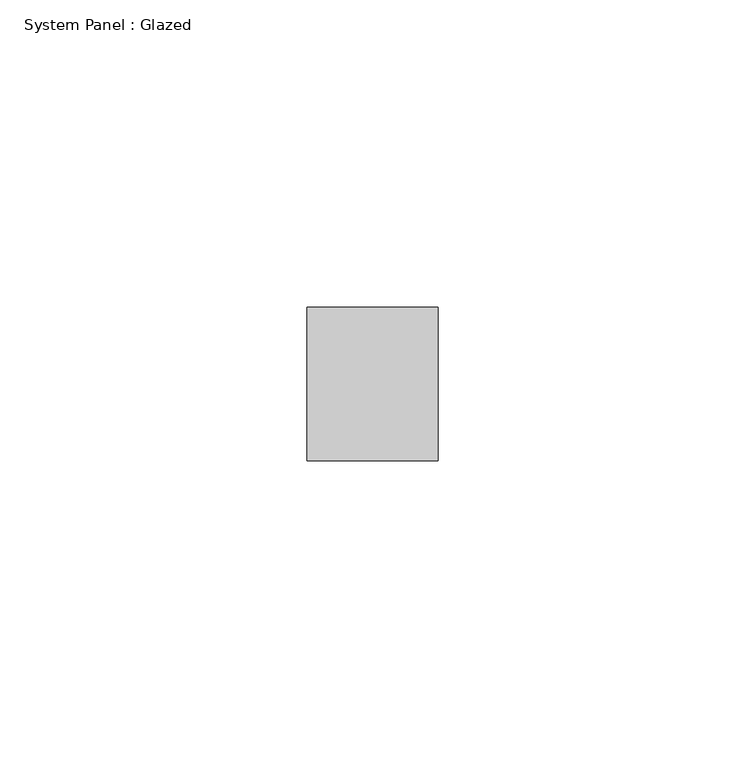
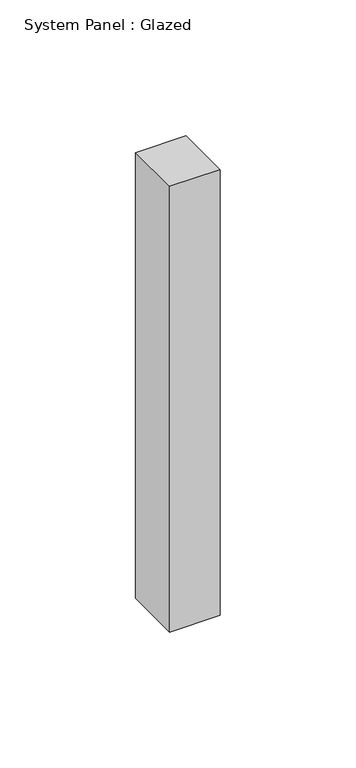
"""IFC4 building model written with IfcOpenShell, lengths in millimetres: plate geometry, System Panel : Glazed."""

import ifcopenshell
import ifcopenshell.guid

model = None  # the IFC model being written
_history = None  # IfcOwnerHistory: only IFC2X3 demands one
_inside = {}  # id of a spatial element -> (the spatial element, [elements in it])
_under = {}  # id of a project, library or spatial element -> (it, [spatial elements below it])
_declared = {}  # id of a project -> (the project, [libraries it declares])
_typed = {}  # id of a type object -> (the type object, [elements of that type])
_made_of = {}  # id of a material, layer set ... -> (it, [elements and type objects made of it])


def new_model(schema):
    """Start an empty IFC model of exactly this schema.

    Asked for "IFC4X3", IfcOpenShell would pick the latest addendum, in which some entities
    have other attributes; the version numbers below select the first issue.
    IFC2X3 requires an IfcOwnerHistory on every rooted entity: one is made here for all.
    """
    global model, _history
    if schema == "IFC4X3":
        model = ifcopenshell.file(schema_version=(4, 3, 0, 0))
    else:
        model = ifcopenshell.file(schema=schema)
    _inside.clear()
    _under.clear()
    _declared.clear()
    _typed.clear()
    _made_of.clear()
    _history = None
    if model.schema == "IFC2X3":
        org = make("IfcOrganization", Name="unknown")
        user = make(
            "IfcPersonAndOrganization",
            ThePerson=make("IfcPerson", FamilyName="unknown"),
            TheOrganization=org,
        )
        app = make(
            "IfcApplication",
            ApplicationDeveloper=org,
            Version="unknown",
            ApplicationFullName="unknown",
            ApplicationIdentifier="unknown",
        )
        _history = make(
            "IfcOwnerHistory",
            OwningUser=user,
            OwningApplication=app,
            ChangeAction="ADDED",
            CreationDate=0,
        )
    return model


def make(cls, **values):
    """One entity of the class cls with the attributes given. An attribute that is None is left unset."""
    return model.create_entity(
        cls, **{name: value for name, value in values.items() if value is not None}
    )


def rooted(cls, **values):
    """An entity with a GlobalId (a new one), such as an element, a storey or a relation."""
    return make(cls, GlobalId=ifcopenshell.guid.new(), OwnerHistory=_history, **values)


def si_unit(unit_type, name, prefix=None):
    """IfcSIUnit, for example si_unit("LENGTHUNIT", "METRE", prefix="MILLI")."""
    return make("IfcSIUnit", UnitType=unit_type, Prefix=prefix, Name=name)


def assignment(units):
    """IfcUnitAssignment: the units of a project."""
    return None if units is None else make("IfcUnitAssignment", Units=units)


def point(xyz):
    """IfcCartesianPoint."""
    return None if xyz is None else make("IfcCartesianPoint", Coordinates=xyz)


def direction(xyz):
    """IfcDirection."""
    return None if xyz is None else make("IfcDirection", DirectionRatios=xyz)


def frame(location, z_axis=None, x_axis=None):
    """IfcAxis2Placement3D, a coordinate frame: its origin and axes. An axis left out is left unset."""
    return make(
        "IfcAxis2Placement3D",
        Location=point(location),
        Axis=direction(z_axis),
        RefDirection=direction(x_axis),
    )


def origin():
    """The frame at (0, 0, 0) with its axes left unset."""
    return frame((0.0, 0.0, 0.0))


def origin_with_axes():
    """The frame at (0, 0, 0) with the z axis (0, 0, 1) and the x axis (1, 0, 0) written out."""
    return frame((0.0, 0.0, 0.0), z_axis=(0.0, 0.0, 1.0), x_axis=(1.0, 0.0, 0.0))


def place(relative_to, where):
    """IfcLocalPlacement: puts the frame where relative to a parent placement (None: the world)."""
    return make(
        "IfcLocalPlacement", PlacementRelTo=relative_to, RelativePlacement=where
    )


def context(
    kind, dimensions, precision=None, world=None, true_north=None, identifier=None
):
    """IfcGeometricRepresentationContext, for example the 3D "Model" context."""
    return make(
        "IfcGeometricRepresentationContext",
        ContextIdentifier=identifier,
        ContextType=kind,
        CoordinateSpaceDimension=dimensions,
        Precision=precision,
        WorldCoordinateSystem=world,
        TrueNorth=true_north,
    )


def project(units=None, contexts=None):
    """IfcProject with its units and contexts."""
    return rooted(
        "IfcProject",
        Name="project",
        RepresentationContexts=contexts,
        UnitsInContext=assignment(units),
    )


def spatial(cls, under=None, at=None, **own):
    """A site, building, storey or space (cls), placed at a placement, below another one or the project."""
    s = rooted(cls, ObjectPlacement=at, **own)
    if under is not None:
        _under.setdefault(under.id(), (under, []))[1].append(s)
    return s


def polyline(points):
    """IfcPolyline through the points."""
    return make("IfcPolyline", Points=[point(p) for p in points])


def outline(outer, holes=None, kind="AREA"):
    """IfcArbitraryClosedProfileDef: a profile drawn as a closed curve; with holes, ...WithVoids."""
    if holes is None:
        return make("IfcArbitraryClosedProfileDef", ProfileType=kind, OuterCurve=outer)
    return make(
        "IfcArbitraryProfileDefWithVoids",
        ProfileType=kind,
        OuterCurve=outer,
        InnerCurves=holes,
    )


def extrude(swept, where, along, depth):
    """IfcExtrudedAreaSolid: the profile swept, set in the frame where, extruded along a direction by depth."""
    return make(
        "IfcExtrudedAreaSolid",
        SweptArea=swept,
        Position=where,
        ExtrudedDirection=direction(along),
        Depth=depth,
    )


def shape(context_of_items, identifier, shape_type, items):
    """IfcShapeRepresentation: the items that make up one representation, for example the "Body"."""
    return make(
        "IfcShapeRepresentation",
        ContextOfItems=context_of_items,
        RepresentationIdentifier=identifier,
        RepresentationType=shape_type,
        Items=items,
    )


def source(mapping_origin, context_of_items, identifier, shape_type, items):
    """IfcRepresentationMap: a shape defined once, which mapped items show again and again."""
    return make(
        "IfcRepresentationMap",
        MappingOrigin=mapping_origin,
        MappedRepresentation=shape(context_of_items, identifier, shape_type, items),
    )


def transform(
    local_origin,
    x_axis=None,
    y_axis=None,
    z_axis=None,
    scale=None,
    scale2=None,
    scale3=None,
    uniform=True,
):
    """IfcCartesianTransformationOperator3D, or its non-uniform kind. x_axis, y_axis, z_axis: its Axis1, 2, 3."""
    if uniform:
        return make(
            "IfcCartesianTransformationOperator3D",
            Axis1=direction(x_axis),
            Axis2=direction(y_axis),
            LocalOrigin=point(local_origin),
            Scale=scale,
            Axis3=direction(z_axis),
        )
    return make(
        "IfcCartesianTransformationOperator3DnonUniform",
        Axis1=direction(x_axis),
        Axis2=direction(y_axis),
        LocalOrigin=point(local_origin),
        Scale=scale,
        Axis3=direction(z_axis),
        Scale2=scale2,
        Scale3=scale3,
    )


def mapped(mapping_source, mapping_target):
    """IfcMappedItem: shows the shape of a source again, moved by a transform."""
    return make(
        "IfcMappedItem", MappingSource=mapping_source, MappingTarget=mapping_target
    )


def made_of(thing, what):
    """Note that an element or type object is made of a material, layer set ...; save() writes the relation."""
    if what is not None:
        _made_of.setdefault(what.id(), (what, []))[1].append(thing)
    return thing


def element(
    cls,
    number,
    at=None,
    inside=None,
    cuts=None,
    type_object=None,
    material=None,
    context=None,
    identifier="Body",
    shape_type=None,
    held_by="IfcProductDefinitionShape",
    body=None,
    shapes=None,
    **own,
):
    """One element of the class cls, such as IfcWall. Its Tag is "e" and its number.

    at: its placement. inside: the storey or other place that contains it. cuts: it is an
    opening in that element (IfcRelVoidsElement). A single representation is given by context,
    identifier, shape_type and body (its items); several are given by shapes. held_by: the class
    of the entity that holds the representations. save() writes the other relations.
    """
    e = rooted(cls, Tag="e%d" % number, ObjectPlacement=at, **own)
    if body is not None:
        shapes = [shape(context, identifier, shape_type, body)]
    if shapes is not None:
        e.Representation = make(held_by, Representations=shapes)
    if inside is not None:
        _inside.setdefault(inside.id(), (inside, []))[1].append(e)
    if cuts is not None:
        rooted(
            "IfcRelVoidsElement", RelatingBuildingElement=cuts, RelatedOpeningElement=e
        )
    if type_object is not None:
        _typed.setdefault(type_object.id(), (type_object, []))[1].append(e)
    return made_of(e, material)


def aggregate(whole, parts):
    """IfcRelAggregates: a whole, such as a stair, and the parts it consists of."""
    return rooted("IfcRelAggregates", RelatingObject=whole, RelatedObjects=parts)


def save(model, path):
    """Write the relations noted so far, then the file.

    IfcRelAggregates (storeys below a building ...), IfcRelContainedInSpatialStructure (elements
    in a storey), IfcRelDefinesByType, IfcRelAssociatesMaterial and IfcRelDeclares: one each for
    every whole, place, type object, material and project.
    """
    for whole, parts in _under.values():
        aggregate(whole, parts)
    for where, things in _inside.values():
        rooted(
            "IfcRelContainedInSpatialStructure",
            RelatedElements=things,
            RelatingStructure=where,
        )
    for kind, things in _typed.values():
        rooted("IfcRelDefinesByType", RelatedObjects=things, RelatingType=kind)
    for what, things in _made_of.values():
        rooted("IfcRelAssociatesMaterial", RelatedObjects=things, RelatingMaterial=what)
    for by, libraries in _declared.values():
        rooted("IfcRelDeclares", RelatingContext=by, RelatedDefinitions=libraries)
    model.write(path)


def system_panel_glazed_87147500(model_context):
    return source(origin(), model_context, "Body", "SweptSolid", [
        extrude(outline(polyline([(10.6704335, 24.5), (-10.6704335, 24.5), (-10.6704335, 49.5), (10.6704335, 49.5), (10.6704335, 24.5)])), origin_with_axes(), (0.0, 0.0, 1.0), 200.0),
    ])


if __name__ == "__main__":
    model = new_model("IFC4")
    model_context = context("Model", 3, world=origin())
    ifc_project = project(units=[si_unit("LENGTHUNIT", "METRE", prefix="MILLI")], contexts=[model_context])
    site = spatial("IfcSite", under=ifc_project)
    building = spatial("IfcBuilding", under=site)
    placement = place(None, origin())
    system_panel_glazed_shape = system_panel_glazed_87147500(model_context)
    element("IfcPlate", 1, ObjectType="System Panel : Glazed", at=placement, inside=building, context=model_context, shape_type="MappedRepresentation", body=[
        mapped(system_panel_glazed_shape, transform((0.0, 0.0, 0.0), x_axis=(1.0, 0.0, 0.0), y_axis=(0.0, 1.0, 0.0), z_axis=(0.0, 0.0, 1.0))),
    ])
    save(model, "model.ifc")

# Revit data of these elements
# Element 1 (IfcPlate, "System Panel : Glazed")
#   Materials on its faces: "Glass"
# Materials
#   "Glass": class "Glass", colour RGB 218 227 224, transparency 0.85, Description = "Soda Lime Glass", Cost = 0
